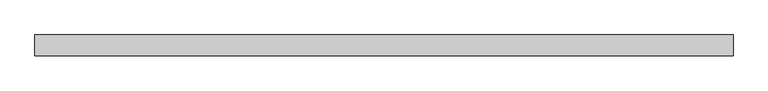
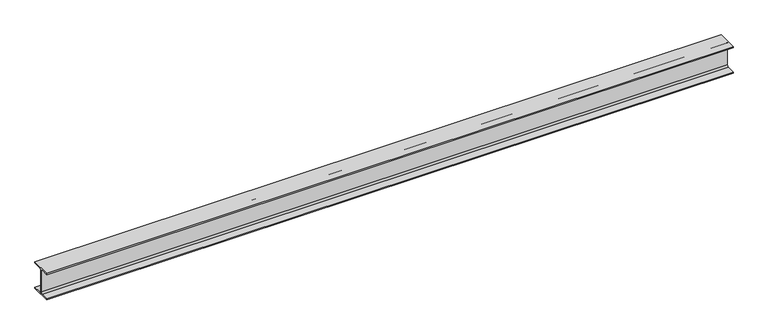
"""IFC4 building model written with IfcOpenShell, lengths in millimetres: beam geometry, 0912_Steel Framing_H-KSD3502 : H_SB_ASB_H-340x250x9x14."""

from ifc_helpers import new_model, si_unit, point, frame, frame_2d, origin, place, context, project, spatial, polyline, circle_curve, trimmed, segment, composite_curve, outline, extrude, source, transform, mapped, element, save


def beam_20af3033(model_context):
    return source(origin(), model_context, "Body", "SweptSolid", [
        extrude(outline(composite_curve([segment(polyline([(125.0, -156.0), (125.0, -170.0), (-125.0, -170.0), (-125.0, -156.0), (-24.5, -156.0)]), True, "CONTINUOUS"), segment(trimmed(circle_curve(frame_2d((-24.5, -136.0)), 20.0), [point((-24.5, -156.0))], [point((-4.5, -136.0))], True, "CARTESIAN"), True, "CONTINUOUS"), segment(polyline([(-4.5, -136.0), (-4.5, 136.0)]), True, "CONTINUOUS"), segment(trimmed(circle_curve(frame_2d((-24.5, 136.0)), 20.0), [point((-4.5, 136.0))], [point((-24.5, 156.0))], True, "CARTESIAN"), True, "CONTINUOUS"), segment(polyline([(-24.5, 156.0), (-125.0, 156.0), (-125.0, 170.0), (125.0, 170.0), (125.0, 156.0), (24.5, 156.0)]), True, "CONTINUOUS"), segment(trimmed(circle_curve(frame_2d((24.5, 136.0)), 20.0), [point((24.5, 156.0))], [point((4.5, 136.0))], True, "CARTESIAN"), True, "CONTINUOUS"), segment(polyline([(4.5, 136.0), (4.5, -136.0)]), True, "CONTINUOUS"), segment(trimmed(circle_curve(frame_2d((24.5, -136.0)), 20.0), [point((4.5, -136.0))], [point((24.5, -156.0))], True, "CARTESIAN"), True, "CONTINUOUS"), segment(polyline([(24.5, -156.0), (125.0, -156.0)]), True, "CONTINUOUS")], self_intersect=False)), frame((-4087.3, 0.0, 0.0), z_axis=(1.0, 0.0, 0.0), x_axis=(0.0, 1.0, 0.0)), (0.0, 0.0, 1.0), 8337.3),
    ])


if __name__ == "__main__":
    model = new_model("IFC4")
    model_context = context("Model", 3, world=origin())
    ifc_project = project(units=[si_unit("LENGTHUNIT", "METRE", prefix="MILLI")], contexts=[model_context])
    site = spatial("IfcSite", under=ifc_project)
    building = spatial("IfcBuilding", under=site)
    placement = place(None, origin())
    beam_shape = beam_20af3033(model_context)
    element("IfcBeam", 1, ObjectType="0912_Steel Framing_H-KSD3502 : H_SB_ASB_H-340x250x9x14", at=placement, inside=building, context=model_context, shape_type="MappedRepresentation", body=[
        mapped(beam_shape, transform((0.0, 0.0, 0.0), x_axis=(1.0, 0.0, 0.0), y_axis=(0.0, 1.0, 0.0), z_axis=(0.0, 0.0, 1.0))),
    ])
    save(model, "model.ifc")

# Revit data of these elements
# Type "0912_Steel Framing_H-KSD3502 : H_SB_ASB_H-340x250x9x14"
#   H_WM Code_1 = "S01AA002-00001 | Main Steel Structure Fabrication Work | Shelter/Building | Medium Steel - Standard (90KG/M>Weight≥30KG/M) | Material: (   )"
#   H_WM Code_2 = "S03AA028-00001 | Main Steel Structure Erection Work | Shelter/Building | Medium Steel (90KG/M>Weight≥30KG/M) | Material: (   )"
#   H_WM Code_3 = "S01AA010-00001 | Main Steel Structure Fabrication Work | Shelter/Building | Steel Painting/Coating | for Non-Fireproofed Steel Surface, Surface Preparation, Primer, Second & Final Coat | Material: (   )"
#   H_Q'ty Cal Type Tag = "SB-Q2"
#   Width = 25.0 cm
#   Web Thickness = 0.9 cm
#   Web Fillet = 2.0 cm
#   Warping Constant = 969000.0 cm⁶
#   W = 0
#   Torsional Moment of Inertia = 53.6551 cm⁴
#   Section Area = 101.5 cm²
#   Plastic Modulus weak axis = 447.0 cm³
#   Plastic Modulus strong axis = 1410.0 cm³
#   Perimeter = 1.63 m²/m
#   Nominal Weight = 79.70 kgf/m
#   Moment of Inertia weak axis = 3650.00 cm⁴
#   Moment of Inertia strong axis = 21700.00 cm⁴
#   Height = 34.0 cm
#   Flange Thickness = 1.4 cm
#   Elastic Modulus weak axis = 292.0 cm³
#   Elastic Modulus strong axis = 1280.0 cm³
#   Centroid Vertical = 17.0 cm
#   Centroid Horizontal = 12.5 cm
#   Ix = 217000000
#   Length [instance default] = 1.5240 m
#   Zx = 1410000
#   b = 0.2500 m
#   h = 0.3400 m
#   r = 0.0200 m
#   s = 0.0090 m
#   t = 0.0140 m
#   A = 0.01015 m²
#   Structural Material [instance default] = Steel, 45-345
#   Assembly Code = ""
# Element 1 (IfcBeam, "0912_Steel Framing_H-KSD3502 : H_SB_ASB_H-340x250x9x14")
#   Structural Material = none
# Materials
#   "Steel, 45-345": class "Metal", colour RGB 189 187 185, transparency 0, Description = "Steel 345 MPa", Cost = 0
